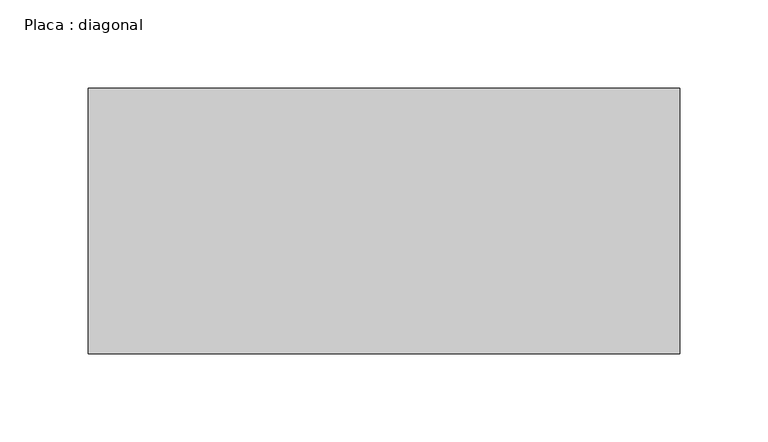
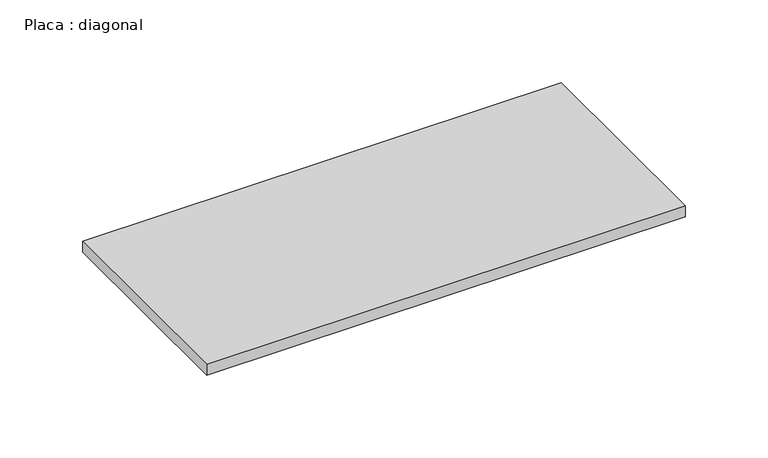
"""IFC4 building model written with IfcOpenShell, lengths in millimetres: beam geometry, Placa : diagonal."""

from ifc_helpers import new_model, si_unit, frame, origin, place, context, project, spatial, polyline, outline, extrude, source, transform, mapped, element, save


def placa_diagonal_30fa4039(model_context):
    return source(origin(), model_context, "Body", "SweptSolid", [
        extrude(outline(polyline([(167.0675386, 75.0), (167.0675386, -75.0), (-167.4240159, -75.0), (-167.4240159, 75.0), (167.0675386, 75.0)])), frame((0.0, 0.0, -4.0), z_axis=(0.0, 0.0, 1.0), x_axis=(1.0, 0.0, 0.0)), (0.0, 0.0, 1.0), 8.0),
    ])


if __name__ == "__main__":
    model = new_model("IFC4")
    model_context = context("Model", 3, world=origin())
    ifc_project = project(units=[si_unit("LENGTHUNIT", "METRE", prefix="MILLI")], contexts=[model_context])
    site = spatial("IfcSite", under=ifc_project)
    building = spatial("IfcBuilding", under=site)
    placement = place(None, origin())
    placa_diagonal_shape = placa_diagonal_30fa4039(model_context)
    element("IfcBeam", 1, ObjectType="Placa : diagonal", at=placement, inside=building, context=model_context, shape_type="MappedRepresentation", body=[
        mapped(placa_diagonal_shape, transform((0.0, 0.0, 0.0), x_axis=(1.0, 0.0, 0.0), y_axis=(0.0, 1.0, 0.0), z_axis=(0.0, 0.0, 1.0))),
    ])
    save(model, "model.ifc")

# Revit data of these elements
# Type "Placa : diagonal"
#   W = 0
#   Length [instance default] = 1.50 m
#   b = 0.15 m
#   d = 0.008 m
#   A = 0 m²
#   Structural Material [instance default] = Aço, 45-345
# Element 1 (IfcBeam, "Placa : diagonal")
#   Materials on its faces: "Aço, 45-345"
# Materials
#   "Aço, 45-345": class "Metal", colour RGB 247 247 247, transparency 0, Description = "Aço 345 MPa", Cost = 0
